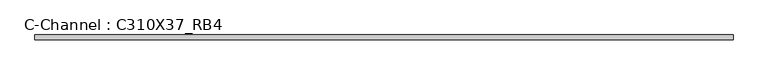
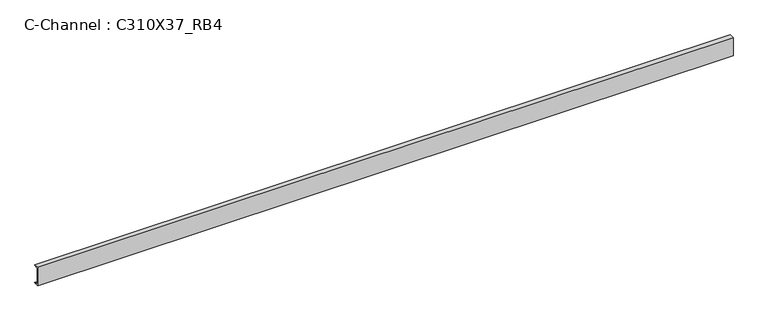
"""IFC4 building model written with IfcOpenShell, lengths in millimetres: beam geometry, C-Channel : C310X37_RB4."""

import ifcopenshell
import ifcopenshell.guid

model = None  # the IFC model being written
_history = None  # IfcOwnerHistory: only IFC2X3 demands one
_inside = {}  # id of a spatial element -> (the spatial element, [elements in it])
_under = {}  # id of a project, library or spatial element -> (it, [spatial elements below it])
_declared = {}  # id of a project -> (the project, [libraries it declares])
_typed = {}  # id of a type object -> (the type object, [elements of that type])
_made_of = {}  # id of a material, layer set ... -> (it, [elements and type objects made of it])


def new_model(schema):
    """Start an empty IFC model of exactly this schema.

    Asked for "IFC4X3", IfcOpenShell would pick the latest addendum, in which some entities
    have other attributes; the version numbers below select the first issue.
    IFC2X3 requires an IfcOwnerHistory on every rooted entity: one is made here for all.
    """
    global model, _history
    if schema == "IFC4X3":
        model = ifcopenshell.file(schema_version=(4, 3, 0, 0))
    else:
        model = ifcopenshell.file(schema=schema)
    _inside.clear()
    _under.clear()
    _declared.clear()
    _typed.clear()
    _made_of.clear()
    _history = None
    if model.schema == "IFC2X3":
        org = make("IfcOrganization", Name="unknown")
        user = make(
            "IfcPersonAndOrganization",
            ThePerson=make("IfcPerson", FamilyName="unknown"),
            TheOrganization=org,
        )
        app = make(
            "IfcApplication",
            ApplicationDeveloper=org,
            Version="unknown",
            ApplicationFullName="unknown",
            ApplicationIdentifier="unknown",
        )
        _history = make(
            "IfcOwnerHistory",
            OwningUser=user,
            OwningApplication=app,
            ChangeAction="ADDED",
            CreationDate=0,
        )
    return model


def make(cls, **values):
    """One entity of the class cls with the attributes given. An attribute that is None is left unset."""
    return model.create_entity(
        cls, **{name: value for name, value in values.items() if value is not None}
    )


def rooted(cls, **values):
    """An entity with a GlobalId (a new one), such as an element, a storey or a relation."""
    return make(cls, GlobalId=ifcopenshell.guid.new(), OwnerHistory=_history, **values)


def si_unit(unit_type, name, prefix=None):
    """IfcSIUnit, for example si_unit("LENGTHUNIT", "METRE", prefix="MILLI")."""
    return make("IfcSIUnit", UnitType=unit_type, Prefix=prefix, Name=name)


def assignment(units):
    """IfcUnitAssignment: the units of a project."""
    return None if units is None else make("IfcUnitAssignment", Units=units)


def point(xyz):
    """IfcCartesianPoint."""
    return None if xyz is None else make("IfcCartesianPoint", Coordinates=xyz)


def direction(xyz):
    """IfcDirection."""
    return None if xyz is None else make("IfcDirection", DirectionRatios=xyz)


def frame(location, z_axis=None, x_axis=None):
    """IfcAxis2Placement3D, a coordinate frame: its origin and axes. An axis left out is left unset."""
    return make(
        "IfcAxis2Placement3D",
        Location=point(location),
        Axis=direction(z_axis),
        RefDirection=direction(x_axis),
    )


def frame_2d(location, x_axis=None):
    """IfcAxis2Placement2D, a coordinate frame in the plane: its origin and x axis."""
    return make(
        "IfcAxis2Placement2D", Location=point(location), RefDirection=direction(x_axis)
    )


def origin():
    """The frame at (0, 0, 0) with its axes left unset."""
    return frame((0.0, 0.0, 0.0))


def place(relative_to, where):
    """IfcLocalPlacement: puts the frame where relative to a parent placement (None: the world)."""
    return make(
        "IfcLocalPlacement", PlacementRelTo=relative_to, RelativePlacement=where
    )


def context(
    kind, dimensions, precision=None, world=None, true_north=None, identifier=None
):
    """IfcGeometricRepresentationContext, for example the 3D "Model" context."""
    return make(
        "IfcGeometricRepresentationContext",
        ContextIdentifier=identifier,
        ContextType=kind,
        CoordinateSpaceDimension=dimensions,
        Precision=precision,
        WorldCoordinateSystem=world,
        TrueNorth=true_north,
    )


def project(units=None, contexts=None):
    """IfcProject with its units and contexts."""
    return rooted(
        "IfcProject",
        Name="project",
        RepresentationContexts=contexts,
        UnitsInContext=assignment(units),
    )


def spatial(cls, under=None, at=None, **own):
    """A site, building, storey or space (cls), placed at a placement, below another one or the project."""
    s = rooted(cls, ObjectPlacement=at, **own)
    if under is not None:
        _under.setdefault(under.id(), (under, []))[1].append(s)
    return s


def polyline(points):
    """IfcPolyline through the points."""
    return make("IfcPolyline", Points=[point(p) for p in points])


def circle_curve(where, radius):
    """IfcCircle in the frame where."""
    return make("IfcCircle", Position=where, Radius=radius)


def trimmed(basis, trim1, trim2, sense, master):
    """IfcTrimmedCurve: the piece of a basis curve between two trims."""
    return make(
        "IfcTrimmedCurve",
        BasisCurve=basis,
        Trim1=trim1,
        Trim2=trim2,
        SenseAgreement=sense,
        MasterRepresentation=master,
    )


def segment(curve, same_sense, transition):
    """IfcCompositeCurveSegment."""
    return make(
        "IfcCompositeCurveSegment",
        Transition=transition,
        SameSense=same_sense,
        ParentCurve=curve,
    )


def composite_curve(segments, self_intersect=None):
    """IfcCompositeCurve: segments joined end to end."""
    return make("IfcCompositeCurve", Segments=segments, SelfIntersect=self_intersect)


def outline(outer, holes=None, kind="AREA"):
    """IfcArbitraryClosedProfileDef: a profile drawn as a closed curve; with holes, ...WithVoids."""
    if holes is None:
        return make("IfcArbitraryClosedProfileDef", ProfileType=kind, OuterCurve=outer)
    return make(
        "IfcArbitraryProfileDefWithVoids",
        ProfileType=kind,
        OuterCurve=outer,
        InnerCurves=holes,
    )


def extrude(swept, where, along, depth):
    """IfcExtrudedAreaSolid: the profile swept, set in the frame where, extruded along a direction by depth."""
    return make(
        "IfcExtrudedAreaSolid",
        SweptArea=swept,
        Position=where,
        ExtrudedDirection=direction(along),
        Depth=depth,
    )


def shape(context_of_items, identifier, shape_type, items):
    """IfcShapeRepresentation: the items that make up one representation, for example the "Body"."""
    return make(
        "IfcShapeRepresentation",
        ContextOfItems=context_of_items,
        RepresentationIdentifier=identifier,
        RepresentationType=shape_type,
        Items=items,
    )


def source(mapping_origin, context_of_items, identifier, shape_type, items):
    """IfcRepresentationMap: a shape defined once, which mapped items show again and again."""
    return make(
        "IfcRepresentationMap",
        MappingOrigin=mapping_origin,
        MappedRepresentation=shape(context_of_items, identifier, shape_type, items),
    )


def transform(
    local_origin,
    x_axis=None,
    y_axis=None,
    z_axis=None,
    scale=None,
    scale2=None,
    scale3=None,
    uniform=True,
):
    """IfcCartesianTransformationOperator3D, or its non-uniform kind. x_axis, y_axis, z_axis: its Axis1, 2, 3."""
    if uniform:
        return make(
            "IfcCartesianTransformationOperator3D",
            Axis1=direction(x_axis),
            Axis2=direction(y_axis),
            LocalOrigin=point(local_origin),
            Scale=scale,
            Axis3=direction(z_axis),
        )
    return make(
        "IfcCartesianTransformationOperator3DnonUniform",
        Axis1=direction(x_axis),
        Axis2=direction(y_axis),
        LocalOrigin=point(local_origin),
        Scale=scale,
        Axis3=direction(z_axis),
        Scale2=scale2,
        Scale3=scale3,
    )


def mapped(mapping_source, mapping_target):
    """IfcMappedItem: shows the shape of a source again, moved by a transform."""
    return make(
        "IfcMappedItem", MappingSource=mapping_source, MappingTarget=mapping_target
    )


def made_of(thing, what):
    """Note that an element or type object is made of a material, layer set ...; save() writes the relation."""
    if what is not None:
        _made_of.setdefault(what.id(), (what, []))[1].append(thing)
    return thing


def element(
    cls,
    number,
    at=None,
    inside=None,
    cuts=None,
    type_object=None,
    material=None,
    context=None,
    identifier="Body",
    shape_type=None,
    held_by="IfcProductDefinitionShape",
    body=None,
    shapes=None,
    **own,
):
    """One element of the class cls, such as IfcWall. Its Tag is "e" and its number.

    at: its placement. inside: the storey or other place that contains it. cuts: it is an
    opening in that element (IfcRelVoidsElement). A single representation is given by context,
    identifier, shape_type and body (its items); several are given by shapes. held_by: the class
    of the entity that holds the representations. save() writes the other relations.
    """
    e = rooted(cls, Tag="e%d" % number, ObjectPlacement=at, **own)
    if body is not None:
        shapes = [shape(context, identifier, shape_type, body)]
    if shapes is not None:
        e.Representation = make(held_by, Representations=shapes)
    if inside is not None:
        _inside.setdefault(inside.id(), (inside, []))[1].append(e)
    if cuts is not None:
        rooted(
            "IfcRelVoidsElement", RelatingBuildingElement=cuts, RelatedOpeningElement=e
        )
    if type_object is not None:
        _typed.setdefault(type_object.id(), (type_object, []))[1].append(e)
    return made_of(e, material)


def aggregate(whole, parts):
    """IfcRelAggregates: a whole, such as a stair, and the parts it consists of."""
    return rooted("IfcRelAggregates", RelatingObject=whole, RelatedObjects=parts)


def save(model, path):
    """Write the relations noted so far, then the file.

    IfcRelAggregates (storeys below a building ...), IfcRelContainedInSpatialStructure (elements
    in a storey), IfcRelDefinesByType, IfcRelAssociatesMaterial and IfcRelDeclares: one each for
    every whole, place, type object, material and project.
    """
    for whole, parts in _under.values():
        aggregate(whole, parts)
    for where, things in _inside.values():
        rooted(
            "IfcRelContainedInSpatialStructure",
            RelatedElements=things,
            RelatingStructure=where,
        )
    for kind, things in _typed.values():
        rooted("IfcRelDefinesByType", RelatedObjects=things, RelatingType=kind)
    for what, things in _made_of.values():
        rooted("IfcRelAssociatesMaterial", RelatedObjects=things, RelatingMaterial=what)
    for by, libraries in _declared.values():
        rooted("IfcRelDeclares", RelatingContext=by, RelatedDefinitions=libraries)
    model.write(path)


def c_channel_c310x37_rb4_7d0df206(model_context):
    return source(origin(), model_context, "Body", "SweptSolid", [
        extrude(outline(composite_curve([segment(polyline([(-17.1196, 152.4), (60.3504, 152.4)]), True, "CONTINUOUS"), segment(trimmed(circle_curve(frame_2d((47.625, 152.4)), 12.7254), [point((60.3504, 152.4))], [point((47.625, 139.6746))], False, "CARTESIAN"), True, "CONTINUOUS"), segment(polyline([(47.625, 139.6746), (-7.2898, 130.9769501), (-7.2898, -130.9769501), (47.625, -139.6746)]), True, "CONTINUOUS"), segment(trimmed(circle_curve(frame_2d((47.625, -152.4)), 12.7254), [point((47.625, -139.6746))], [point((60.3504, -152.4))], False, "CARTESIAN"), True, "CONTINUOUS"), segment(polyline([(60.3504, -152.4), (-17.1196, -152.4), (-17.1196, 152.4)]), True, "CONTINUOUS")], self_intersect=False)), frame((-5530.0, 0.0, 0.0), z_axis=(1.0, 0.0, 0.0), x_axis=(0.0, 1.0, 0.0)), (0.0, 0.0, 1.0), 11060.0),
    ])


if __name__ == "__main__":
    model = new_model("IFC4")
    model_context = context("Model", 3, world=origin())
    ifc_project = project(units=[si_unit("LENGTHUNIT", "METRE", prefix="MILLI")], contexts=[model_context])
    site = spatial("IfcSite", under=ifc_project)
    building = spatial("IfcBuilding", under=site)
    placement = place(None, origin())
    c_channel_c310x37_rb4_shape = c_channel_c310x37_rb4_7d0df206(model_context)
    element("IfcBeam", 1, ObjectType="C-Channel : C310X37_RB4", at=placement, inside=building, context=model_context, shape_type="MappedRepresentation", body=[
        mapped(c_channel_c310x37_rb4_shape, transform((0.0, 0.0, 0.0), x_axis=(1.0, 0.0, 0.0), y_axis=(0.0, 1.0, 0.0), z_axis=(0.0, 0.0, 1.0))),
    ])
    save(model, "model.ifc")

# Revit data of these elements
# Type "C-Channel : C310X37_RB4"
#   Assembly Code = "B10"
#   W = 25
#   Length [instance default] = 1524 mm
#   bf = 77.47 mm
#   d = 304.8 mm
#   tf = 12.725 mm
#   tw = 9.83 mm
#   x = 17.12 mm
#   A = 0.00473547 m²
#   Structural Material [instance default] = Steel ASTM A36
# Element 1 (IfcBeam, "C-Channel : C310X37_RB4")
#   Structural Material = Steel ASTM A992
#   Materials on its faces: "Steel ASTM A992"
# Materials
#   "Steel ASTM A36": class "Metal", colour RGB 199 199 199, transparency 0, Description = "Structural steel, ASTM A36 Grade B, mill finish", Cost = 0
#   "Steel ASTM A992": class "Metal", colour RGB 199 199 199, transparency 0, Description = "Structural steel 50ksi", Cost = 0
